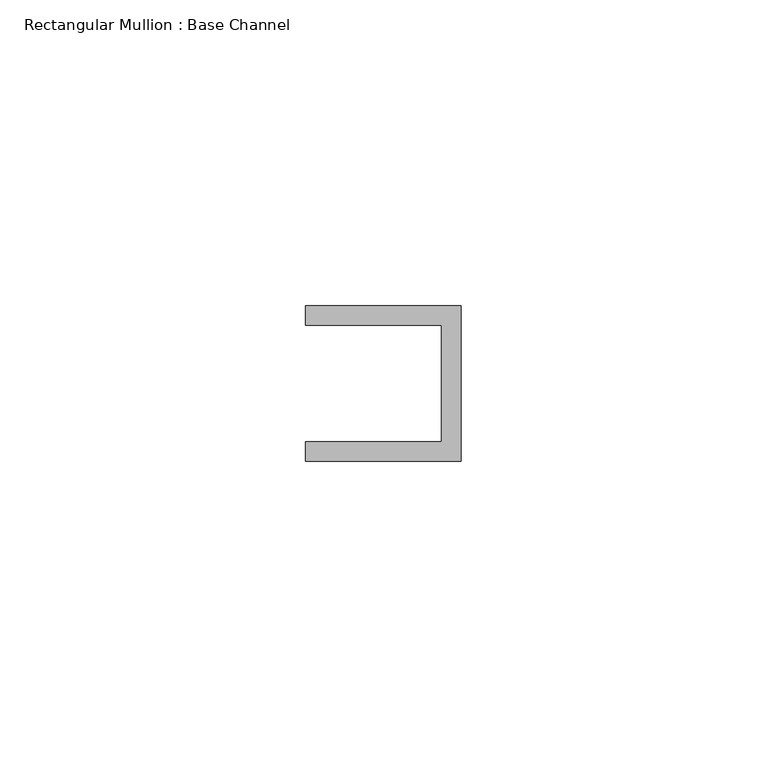
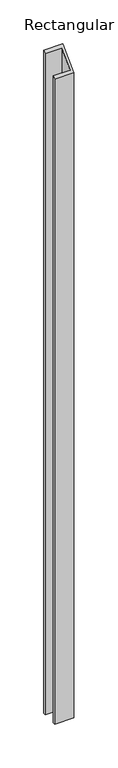
"""IFC4 building model written with IfcOpenShell, lengths in millimetres: member geometry, Rectangular Mullion : Base Channel."""

from ifc_helpers import new_model, si_unit, origin, place, context, project, spatial, faceted_brep, source, transform, mapped, element, save


def rectangular_mullion_base_channel_ca78ccdb(model_context):
    return source(origin(), model_context, "Body", "Brep", [
        faceted_brep([(0.0, -12.7, -914.4000003), (-25.4, -12.7, -914.4000003), (-25.4, -9.525, -914.4000003), (-3.175, -9.525, -914.4000003), (-3.175, 9.525, -914.4000003), (-25.4, 9.525, -914.4000003), (-25.4, 12.7, -914.4000003), (0.0, 12.7, -914.4000003), (0.0, 12.7, 12.7), (0.0, -12.7, -12.7), (-25.4, 12.7, 12.7), (-25.4, 9.525, 9.525), (-3.175, 9.525, 9.525), (-3.175, -9.525, -9.525), (-25.4, -9.525, -9.525), (-25.4, -12.7, -12.7)], [[[0, 1, 2, 3, 4, 5, 6, 7]], [[8, 9, 0, 7]], [[10, 8, 7, 6]], [[11, 10, 6, 5]], [[12, 11, 5, 4]], [[13, 12, 4, 3]], [[14, 13, 3, 2]], [[15, 14, 2, 1]], [[9, 15, 1, 0]], [[9, 8, 10, 11, 12, 13, 14, 15]]]),
    ])


if __name__ == "__main__":
    model = new_model("IFC4")
    model_context = context("Model", 3, world=origin())
    ifc_project = project(units=[si_unit("LENGTHUNIT", "METRE", prefix="MILLI")], contexts=[model_context])
    site = spatial("IfcSite", under=ifc_project)
    building = spatial("IfcBuilding", under=site)
    placement = place(None, origin())
    rectangular_mullion_base_channel_shape = rectangular_mullion_base_channel_ca78ccdb(model_context)
    element("IfcMember", 1, ObjectType="Rectangular Mullion : Base Channel", at=placement, inside=building, context=model_context, shape_type="MappedRepresentation", body=[
        mapped(rectangular_mullion_base_channel_shape, transform((0.0, 0.0, 0.0), x_axis=(1.0, 0.0, 0.0), y_axis=(0.0, 1.0, 0.0), z_axis=(0.0, 0.0, 1.0))),
    ])
    save(model, "model.ifc")

# Revit data of these elements
# Type "Rectangular Mullion : Base Channel"
#   built-in parameter 1007322 = 0.0833333 (stored number, unit not read)
#   built-in parameter 1007321 = 0.0416667 (stored number, unit not read)
#   built-in parameter 1007320 = -0.03125 (stored number, unit not read)
# Element 1 (IfcMember, "Rectangular Mullion : Base Channel")
#   Materials on its faces: "ALUM"
# Materials
#   "ALUM": class "Generic", colour RGB 157 157 157, transparency 0, Cost = 0
